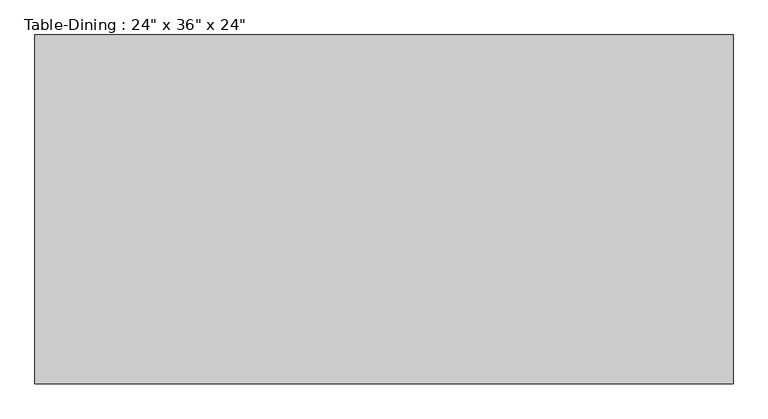
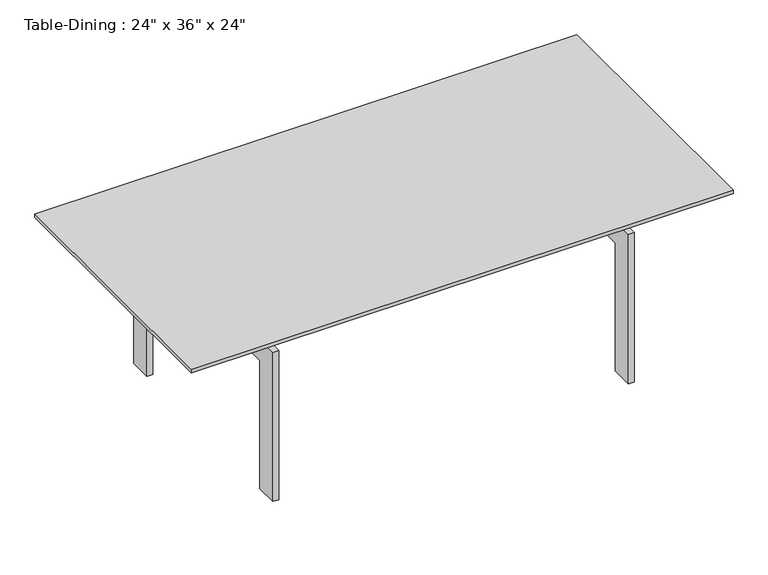
"""IFC4 building model written with IfcOpenShell, lengths in millimetres: furniture geometry."""

import ifcopenshell
import ifcopenshell.guid

model = None  # the IFC model being written
_history = None  # IfcOwnerHistory: only IFC2X3 demands one
_inside = {}  # id of a spatial element -> (the spatial element, [elements in it])
_under = {}  # id of a project, library or spatial element -> (it, [spatial elements below it])
_declared = {}  # id of a project -> (the project, [libraries it declares])
_typed = {}  # id of a type object -> (the type object, [elements of that type])
_made_of = {}  # id of a material, layer set ... -> (it, [elements and type objects made of it])


def new_model(schema):
    """Start an empty IFC model of exactly this schema.

    Asked for "IFC4X3", IfcOpenShell would pick the latest addendum, in which some entities
    have other attributes; the version numbers below select the first issue.
    IFC2X3 requires an IfcOwnerHistory on every rooted entity: one is made here for all.
    """
    global model, _history
    if schema == "IFC4X3":
        model = ifcopenshell.file(schema_version=(4, 3, 0, 0))
    else:
        model = ifcopenshell.file(schema=schema)
    _inside.clear()
    _under.clear()
    _declared.clear()
    _typed.clear()
    _made_of.clear()
    _history = None
    if model.schema == "IFC2X3":
        org = make("IfcOrganization", Name="unknown")
        user = make(
            "IfcPersonAndOrganization",
            ThePerson=make("IfcPerson", FamilyName="unknown"),
            TheOrganization=org,
        )
        app = make(
            "IfcApplication",
            ApplicationDeveloper=org,
            Version="unknown",
            ApplicationFullName="unknown",
            ApplicationIdentifier="unknown",
        )
        _history = make(
            "IfcOwnerHistory",
            OwningUser=user,
            OwningApplication=app,
            ChangeAction="ADDED",
            CreationDate=0,
        )
    return model


def make(cls, **values):
    """One entity of the class cls with the attributes given. An attribute that is None is left unset."""
    return model.create_entity(
        cls, **{name: value for name, value in values.items() if value is not None}
    )


def rooted(cls, **values):
    """An entity with a GlobalId (a new one), such as an element, a storey or a relation."""
    return make(cls, GlobalId=ifcopenshell.guid.new(), OwnerHistory=_history, **values)


def si_unit(unit_type, name, prefix=None):
    """IfcSIUnit, for example si_unit("LENGTHUNIT", "METRE", prefix="MILLI")."""
    return make("IfcSIUnit", UnitType=unit_type, Prefix=prefix, Name=name)


def assignment(units):
    """IfcUnitAssignment: the units of a project."""
    return None if units is None else make("IfcUnitAssignment", Units=units)


def point(xyz):
    """IfcCartesianPoint."""
    return None if xyz is None else make("IfcCartesianPoint", Coordinates=xyz)


def direction(xyz):
    """IfcDirection."""
    return None if xyz is None else make("IfcDirection", DirectionRatios=xyz)


def frame(location, z_axis=None, x_axis=None):
    """IfcAxis2Placement3D, a coordinate frame: its origin and axes. An axis left out is left unset."""
    return make(
        "IfcAxis2Placement3D",
        Location=point(location),
        Axis=direction(z_axis),
        RefDirection=direction(x_axis),
    )


def origin():
    """The frame at (0, 0, 0) with its axes left unset."""
    return frame((0.0, 0.0, 0.0))


def place(relative_to, where):
    """IfcLocalPlacement: puts the frame where relative to a parent placement (None: the world)."""
    return make(
        "IfcLocalPlacement", PlacementRelTo=relative_to, RelativePlacement=where
    )


def context(
    kind, dimensions, precision=None, world=None, true_north=None, identifier=None
):
    """IfcGeometricRepresentationContext, for example the 3D "Model" context."""
    return make(
        "IfcGeometricRepresentationContext",
        ContextIdentifier=identifier,
        ContextType=kind,
        CoordinateSpaceDimension=dimensions,
        Precision=precision,
        WorldCoordinateSystem=world,
        TrueNorth=true_north,
    )


def project(units=None, contexts=None):
    """IfcProject with its units and contexts."""
    return rooted(
        "IfcProject",
        Name="project",
        RepresentationContexts=contexts,
        UnitsInContext=assignment(units),
    )


def spatial(cls, under=None, at=None, **own):
    """A site, building, storey or space (cls), placed at a placement, below another one or the project."""
    s = rooted(cls, ObjectPlacement=at, **own)
    if under is not None:
        _under.setdefault(under.id(), (under, []))[1].append(s)
    return s


def polyline(points):
    """IfcPolyline through the points."""
    return make("IfcPolyline", Points=[point(p) for p in points])


def outline(outer, holes=None, kind="AREA"):
    """IfcArbitraryClosedProfileDef: a profile drawn as a closed curve; with holes, ...WithVoids."""
    if holes is None:
        return make("IfcArbitraryClosedProfileDef", ProfileType=kind, OuterCurve=outer)
    return make(
        "IfcArbitraryProfileDefWithVoids",
        ProfileType=kind,
        OuterCurve=outer,
        InnerCurves=holes,
    )


def extrude(swept, where, along, depth):
    """IfcExtrudedAreaSolid: the profile swept, set in the frame where, extruded along a direction by depth."""
    return make(
        "IfcExtrudedAreaSolid",
        SweptArea=swept,
        Position=where,
        ExtrudedDirection=direction(along),
        Depth=depth,
    )


def shape(context_of_items, identifier, shape_type, items):
    """IfcShapeRepresentation: the items that make up one representation, for example the "Body"."""
    return make(
        "IfcShapeRepresentation",
        ContextOfItems=context_of_items,
        RepresentationIdentifier=identifier,
        RepresentationType=shape_type,
        Items=items,
    )


def source(mapping_origin, context_of_items, identifier, shape_type, items):
    """IfcRepresentationMap: a shape defined once, which mapped items show again and again."""
    return make(
        "IfcRepresentationMap",
        MappingOrigin=mapping_origin,
        MappedRepresentation=shape(context_of_items, identifier, shape_type, items),
    )


def transform(
    local_origin,
    x_axis=None,
    y_axis=None,
    z_axis=None,
    scale=None,
    scale2=None,
    scale3=None,
    uniform=True,
):
    """IfcCartesianTransformationOperator3D, or its non-uniform kind. x_axis, y_axis, z_axis: its Axis1, 2, 3."""
    if uniform:
        return make(
            "IfcCartesianTransformationOperator3D",
            Axis1=direction(x_axis),
            Axis2=direction(y_axis),
            LocalOrigin=point(local_origin),
            Scale=scale,
            Axis3=direction(z_axis),
        )
    return make(
        "IfcCartesianTransformationOperator3DnonUniform",
        Axis1=direction(x_axis),
        Axis2=direction(y_axis),
        LocalOrigin=point(local_origin),
        Scale=scale,
        Axis3=direction(z_axis),
        Scale2=scale2,
        Scale3=scale3,
    )


def mapped(mapping_source, mapping_target):
    """IfcMappedItem: shows the shape of a source again, moved by a transform."""
    return make(
        "IfcMappedItem", MappingSource=mapping_source, MappingTarget=mapping_target
    )


def made_of(thing, what):
    """Note that an element or type object is made of a material, layer set ...; save() writes the relation."""
    if what is not None:
        _made_of.setdefault(what.id(), (what, []))[1].append(thing)
    return thing


def element(
    cls,
    number,
    at=None,
    inside=None,
    cuts=None,
    type_object=None,
    material=None,
    context=None,
    identifier="Body",
    shape_type=None,
    held_by="IfcProductDefinitionShape",
    body=None,
    shapes=None,
    **own,
):
    """One element of the class cls, such as IfcWall. Its Tag is "e" and its number.

    at: its placement. inside: the storey or other place that contains it. cuts: it is an
    opening in that element (IfcRelVoidsElement). A single representation is given by context,
    identifier, shape_type and body (its items); several are given by shapes. held_by: the class
    of the entity that holds the representations. save() writes the other relations.
    """
    e = rooted(cls, Tag="e%d" % number, ObjectPlacement=at, **own)
    if body is not None:
        shapes = [shape(context, identifier, shape_type, body)]
    if shapes is not None:
        e.Representation = make(held_by, Representations=shapes)
    if inside is not None:
        _inside.setdefault(inside.id(), (inside, []))[1].append(e)
    if cuts is not None:
        rooted(
            "IfcRelVoidsElement", RelatingBuildingElement=cuts, RelatedOpeningElement=e
        )
    if type_object is not None:
        _typed.setdefault(type_object.id(), (type_object, []))[1].append(e)
    return made_of(e, material)


def aggregate(whole, parts):
    """IfcRelAggregates: a whole, such as a stair, and the parts it consists of."""
    return rooted("IfcRelAggregates", RelatingObject=whole, RelatedObjects=parts)


def save(model, path):
    """Write the relations noted so far, then the file.

    IfcRelAggregates (storeys below a building ...), IfcRelContainedInSpatialStructure (elements
    in a storey), IfcRelDefinesByType, IfcRelAssociatesMaterial and IfcRelDeclares: one each for
    every whole, place, type object, material and project.
    """
    for whole, parts in _under.values():
        aggregate(whole, parts)
    for where, things in _inside.values():
        rooted(
            "IfcRelContainedInSpatialStructure",
            RelatedElements=things,
            RelatingStructure=where,
        )
    for kind, things in _typed.values():
        rooted("IfcRelDefinesByType", RelatedObjects=things, RelatingType=kind)
    for what, things in _made_of.values():
        rooted("IfcRelAssociatesMaterial", RelatedObjects=things, RelatingMaterial=what)
    for by, libraries in _declared.values():
        rooted("IfcRelDeclares", RelatingContext=by, RelatedDefinitions=libraries)
    model.write(path)


def furniture_5644571f(model_context):
    return source(origin(), model_context, "Body", "SweptSolid", [
        extrude(outline(polyline([(831.0657667, 297.7823857), (831.0657667, 272.3823857), (-794.5342333, 272.3823857), (-794.5342333, 297.7823857), (831.0657667, 297.7823857)])), frame((0.0, 0.0, 533.4), z_axis=(0.0, 0.0, 1.0), x_axis=(1.0, 0.0, 0.0)), (0.0, 0.0, 1.0), 63.5),
        extrude(outline(polyline([(831.0657667, -82.5889222), (831.0657667, -107.9889222), (-794.5342333, -107.9889222), (-794.5342333, -82.5889222), (831.0657667, -82.5889222)])), frame((0.0, 0.0, 533.4), z_axis=(0.0, 0.0, 1.0), x_axis=(1.0, 0.0, 0.0)), (0.0, 0.0, 1.0), 63.5),
        extrude(outline(polyline([(501.6110778, 0.0), (425.4110778, 0.0), (425.4110778, 457.2), (-234.9889222, 457.2), (-234.9889222, 0.0), (-311.1889222, 0.0), (-311.1889222, 533.4), (501.6110778, 533.4), (501.6110778, 0.0)])), frame((608.8157667, 0.0, 0.0), z_axis=(1.0, 0.0, 0.0), x_axis=(0.0, 1.0, 0.0)), (0.0, 0.0, 1.0), 19.05),
        extrude(outline(polyline([(501.6110778, 533.4), (501.6110778, 0.0), (425.4110778, 0.0), (425.4110778, 457.2), (-234.9889222, 457.2), (-234.9889222, 0.0), (-311.1889222, 0.0), (-311.1889222, 533.4), (501.6110778, 533.4)])), frame((-591.3342333, 0.0, 0.0), z_axis=(1.0, 0.0, 0.0), x_axis=(0.0, 1.0, 0.0)), (0.0, 0.0, 1.0), 19.05),
        extrude(outline(polyline([(932.6657667, 552.4110778), (932.6657667, -361.9889222), (-896.1342333, -361.9889222), (-896.1342333, 552.4110778), (932.6657667, 552.4110778)])), frame((0.0, 0.0, 596.9), z_axis=(0.0, 0.0, 1.0), x_axis=(1.0, 0.0, 0.0)), (0.0, 0.0, 1.0), 12.7),
    ])


if __name__ == "__main__":
    model = new_model("IFC4")
    model_context = context("Model", 3, world=origin())
    ifc_project = project(units=[si_unit("LENGTHUNIT", "METRE", prefix="MILLI")], contexts=[model_context])
    site = spatial("IfcSite", under=ifc_project)
    building = spatial("IfcBuilding", under=site)
    placement = place(None, origin())
    furniture_shape = furniture_5644571f(model_context)
    element("IfcFurniture", 1, ObjectType="Table-Dining : 24\" x 36\" x 24\"", at=placement, inside=building, context=model_context, shape_type="MappedRepresentation", body=[
        mapped(furniture_shape, transform((0.0, 0.0, 0.0), x_axis=(1.0, 0.0, 0.0), y_axis=(0.0, 1.0, 0.0), z_axis=(0.0, 0.0, 1.0))),
    ])
    save(model, "model.ifc")

# Revit data of these elements
# Type "Table-Dining : 24\" x 36\" x 24\""
#   Assembly Code = "E2020200"
#   Height = 2' - 0"
#   Length = 6' - 0"
#   Width = 3' - 0"
#   Base Material = Steel, Chrome Plated
#   Top Material = Glass - Clear, Grey
# Element 1 (IfcFurniture, "Table-Dining : 24\" x 36\" x 24\"")
#   Materials on its faces: "Steel, Chrome Plated", "Glass - Clear, Grey"
# Materials
#   "Steel, Chrome Plated": class "Metal", colour RGB 244 244 244, transparency 0, Description = "Chromiuim plated steel", Cost = 0
#   "Glass - Clear, Grey": class "Glass", colour RGB 252 255 255, transparency 0.64
